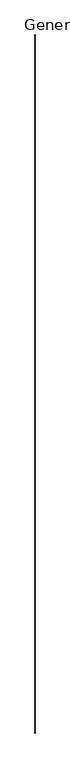
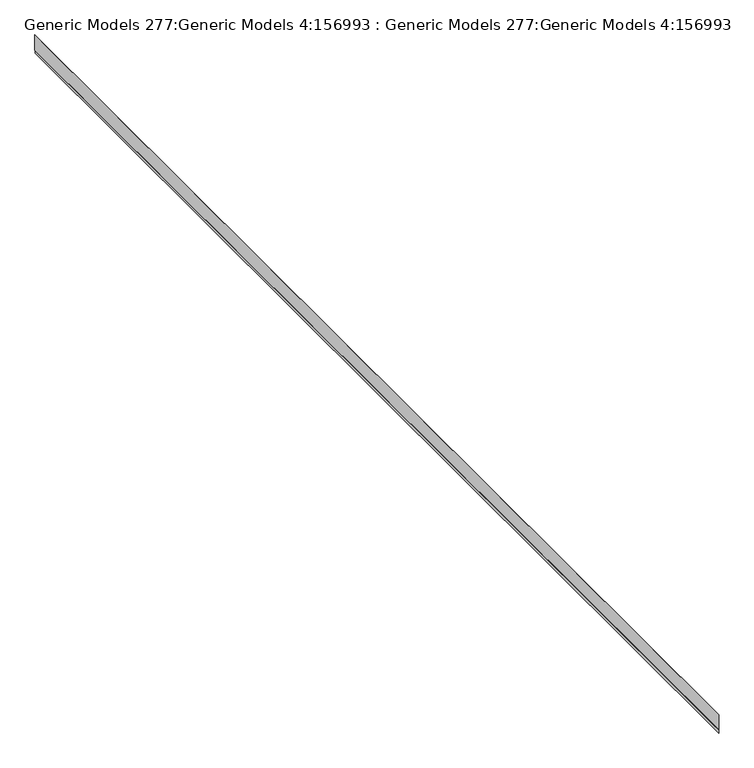
"""IFC4 building model written with IfcOpenShell, lengths in millimetres: proxy geometry, Generic Models 277:Generic Models 4:156993 : Generic Models 277:Generic Models 4:156993."""

import ifcopenshell
import ifcopenshell.guid

model = None  # the IFC model being written
_history = None  # IfcOwnerHistory: only IFC2X3 demands one
_inside = {}  # id of a spatial element -> (the spatial element, [elements in it])
_under = {}  # id of a project, library or spatial element -> (it, [spatial elements below it])
_declared = {}  # id of a project -> (the project, [libraries it declares])
_typed = {}  # id of a type object -> (the type object, [elements of that type])
_made_of = {}  # id of a material, layer set ... -> (it, [elements and type objects made of it])


def new_model(schema):
    """Start an empty IFC model of exactly this schema.

    Asked for "IFC4X3", IfcOpenShell would pick the latest addendum, in which some entities
    have other attributes; the version numbers below select the first issue.
    IFC2X3 requires an IfcOwnerHistory on every rooted entity: one is made here for all.
    """
    global model, _history
    if schema == "IFC4X3":
        model = ifcopenshell.file(schema_version=(4, 3, 0, 0))
    else:
        model = ifcopenshell.file(schema=schema)
    _inside.clear()
    _under.clear()
    _declared.clear()
    _typed.clear()
    _made_of.clear()
    _history = None
    if model.schema == "IFC2X3":
        org = make("IfcOrganization", Name="unknown")
        user = make(
            "IfcPersonAndOrganization",
            ThePerson=make("IfcPerson", FamilyName="unknown"),
            TheOrganization=org,
        )
        app = make(
            "IfcApplication",
            ApplicationDeveloper=org,
            Version="unknown",
            ApplicationFullName="unknown",
            ApplicationIdentifier="unknown",
        )
        _history = make(
            "IfcOwnerHistory",
            OwningUser=user,
            OwningApplication=app,
            ChangeAction="ADDED",
            CreationDate=0,
        )
    return model


def make(cls, **values):
    """One entity of the class cls with the attributes given. An attribute that is None is left unset."""
    return model.create_entity(
        cls, **{name: value for name, value in values.items() if value is not None}
    )


def rooted(cls, **values):
    """An entity with a GlobalId (a new one), such as an element, a storey or a relation."""
    return make(cls, GlobalId=ifcopenshell.guid.new(), OwnerHistory=_history, **values)


def si_unit(unit_type, name, prefix=None):
    """IfcSIUnit, for example si_unit("LENGTHUNIT", "METRE", prefix="MILLI")."""
    return make("IfcSIUnit", UnitType=unit_type, Prefix=prefix, Name=name)


def assignment(units):
    """IfcUnitAssignment: the units of a project."""
    return None if units is None else make("IfcUnitAssignment", Units=units)


def point(xyz):
    """IfcCartesianPoint."""
    return None if xyz is None else make("IfcCartesianPoint", Coordinates=xyz)


def direction(xyz):
    """IfcDirection."""
    return None if xyz is None else make("IfcDirection", DirectionRatios=xyz)


def frame(location, z_axis=None, x_axis=None):
    """IfcAxis2Placement3D, a coordinate frame: its origin and axes. An axis left out is left unset."""
    return make(
        "IfcAxis2Placement3D",
        Location=point(location),
        Axis=direction(z_axis),
        RefDirection=direction(x_axis),
    )


def origin():
    """The frame at (0, 0, 0) with its axes left unset."""
    return frame((0.0, 0.0, 0.0))


def place(relative_to, where):
    """IfcLocalPlacement: puts the frame where relative to a parent placement (None: the world)."""
    return make(
        "IfcLocalPlacement", PlacementRelTo=relative_to, RelativePlacement=where
    )


def context(
    kind, dimensions, precision=None, world=None, true_north=None, identifier=None
):
    """IfcGeometricRepresentationContext, for example the 3D "Model" context."""
    return make(
        "IfcGeometricRepresentationContext",
        ContextIdentifier=identifier,
        ContextType=kind,
        CoordinateSpaceDimension=dimensions,
        Precision=precision,
        WorldCoordinateSystem=world,
        TrueNorth=true_north,
    )


def project(units=None, contexts=None):
    """IfcProject with its units and contexts."""
    return rooted(
        "IfcProject",
        Name="project",
        RepresentationContexts=contexts,
        UnitsInContext=assignment(units),
    )


def spatial(cls, under=None, at=None, **own):
    """A site, building, storey or space (cls), placed at a placement, below another one or the project."""
    s = rooted(cls, ObjectPlacement=at, **own)
    if under is not None:
        _under.setdefault(under.id(), (under, []))[1].append(s)
    return s


def polyline(points):
    """IfcPolyline through the points."""
    return make("IfcPolyline", Points=[point(p) for p in points])


def outline(outer, holes=None, kind="AREA"):
    """IfcArbitraryClosedProfileDef: a profile drawn as a closed curve; with holes, ...WithVoids."""
    if holes is None:
        return make("IfcArbitraryClosedProfileDef", ProfileType=kind, OuterCurve=outer)
    return make(
        "IfcArbitraryProfileDefWithVoids",
        ProfileType=kind,
        OuterCurve=outer,
        InnerCurves=holes,
    )


def extrude(swept, where, along, depth):
    """IfcExtrudedAreaSolid: the profile swept, set in the frame where, extruded along a direction by depth."""
    return make(
        "IfcExtrudedAreaSolid",
        SweptArea=swept,
        Position=where,
        ExtrudedDirection=direction(along),
        Depth=depth,
    )


def shape(context_of_items, identifier, shape_type, items):
    """IfcShapeRepresentation: the items that make up one representation, for example the "Body"."""
    return make(
        "IfcShapeRepresentation",
        ContextOfItems=context_of_items,
        RepresentationIdentifier=identifier,
        RepresentationType=shape_type,
        Items=items,
    )


def source(mapping_origin, context_of_items, identifier, shape_type, items):
    """IfcRepresentationMap: a shape defined once, which mapped items show again and again."""
    return make(
        "IfcRepresentationMap",
        MappingOrigin=mapping_origin,
        MappedRepresentation=shape(context_of_items, identifier, shape_type, items),
    )


def transform(
    local_origin,
    x_axis=None,
    y_axis=None,
    z_axis=None,
    scale=None,
    scale2=None,
    scale3=None,
    uniform=True,
):
    """IfcCartesianTransformationOperator3D, or its non-uniform kind. x_axis, y_axis, z_axis: its Axis1, 2, 3."""
    if uniform:
        return make(
            "IfcCartesianTransformationOperator3D",
            Axis1=direction(x_axis),
            Axis2=direction(y_axis),
            LocalOrigin=point(local_origin),
            Scale=scale,
            Axis3=direction(z_axis),
        )
    return make(
        "IfcCartesianTransformationOperator3DnonUniform",
        Axis1=direction(x_axis),
        Axis2=direction(y_axis),
        LocalOrigin=point(local_origin),
        Scale=scale,
        Axis3=direction(z_axis),
        Scale2=scale2,
        Scale3=scale3,
    )


def mapped(mapping_source, mapping_target):
    """IfcMappedItem: shows the shape of a source again, moved by a transform."""
    return make(
        "IfcMappedItem", MappingSource=mapping_source, MappingTarget=mapping_target
    )


def made_of(thing, what):
    """Note that an element or type object is made of a material, layer set ...; save() writes the relation."""
    if what is not None:
        _made_of.setdefault(what.id(), (what, []))[1].append(thing)
    return thing


def element(
    cls,
    number,
    at=None,
    inside=None,
    cuts=None,
    type_object=None,
    material=None,
    context=None,
    identifier="Body",
    shape_type=None,
    held_by="IfcProductDefinitionShape",
    body=None,
    shapes=None,
    **own,
):
    """One element of the class cls, such as IfcWall. Its Tag is "e" and its number.

    at: its placement. inside: the storey or other place that contains it. cuts: it is an
    opening in that element (IfcRelVoidsElement). A single representation is given by context,
    identifier, shape_type and body (its items); several are given by shapes. held_by: the class
    of the entity that holds the representations. save() writes the other relations.
    """
    e = rooted(cls, Tag="e%d" % number, ObjectPlacement=at, **own)
    if body is not None:
        shapes = [shape(context, identifier, shape_type, body)]
    if shapes is not None:
        e.Representation = make(held_by, Representations=shapes)
    if inside is not None:
        _inside.setdefault(inside.id(), (inside, []))[1].append(e)
    if cuts is not None:
        rooted(
            "IfcRelVoidsElement", RelatingBuildingElement=cuts, RelatedOpeningElement=e
        )
    if type_object is not None:
        _typed.setdefault(type_object.id(), (type_object, []))[1].append(e)
    return made_of(e, material)


def aggregate(whole, parts):
    """IfcRelAggregates: a whole, such as a stair, and the parts it consists of."""
    return rooted("IfcRelAggregates", RelatingObject=whole, RelatedObjects=parts)


def save(model, path):
    """Write the relations noted so far, then the file.

    IfcRelAggregates (storeys below a building ...), IfcRelContainedInSpatialStructure (elements
    in a storey), IfcRelDefinesByType, IfcRelAssociatesMaterial and IfcRelDeclares: one each for
    every whole, place, type object, material and project.
    """
    for whole, parts in _under.values():
        aggregate(whole, parts)
    for where, things in _inside.values():
        rooted(
            "IfcRelContainedInSpatialStructure",
            RelatedElements=things,
            RelatingStructure=where,
        )
    for kind, things in _typed.values():
        rooted("IfcRelDefinesByType", RelatedObjects=things, RelatingType=kind)
    for what, things in _made_of.values():
        rooted("IfcRelAssociatesMaterial", RelatedObjects=things, RelatingMaterial=what)
    for by, libraries in _declared.values():
        rooted("IfcRelDeclares", RelatingContext=by, RelatedDefinitions=libraries)
    model.write(path)


def generic_models_277_generic_models_4_156993_generic_models_47cee2a2(model_context):
    return source(origin(), model_context, "Body", "SweptSolid", [
        extrude(outline(polyline([(6156.5192101, 1597.6373761), (5902.9944211, 1597.6373761), (5897.3527003, 1599.6907945), (5849.785851, 1599.6907945), (5849.785851, 1600.4845445), (5897.4926599, 1600.4845445), (5903.1343806, 1598.4311261), (6156.5192101, 1598.4311261), (6156.5192101, 1597.6373761)])), frame((0.0, -8838.4871142, 0.0), z_axis=(0.0, 1.0, 0.0), x_axis=(0.0, 0.0, 1.0)), (0.0, 0.0, 1.0), 18643.6),
    ])


if __name__ == "__main__":
    model = new_model("IFC4")
    model_context = context("Model", 3, world=origin())
    ifc_project = project(units=[si_unit("LENGTHUNIT", "METRE", prefix="MILLI")], contexts=[model_context])
    site = spatial("IfcSite", under=ifc_project)
    building = spatial("IfcBuilding", under=site)
    placement = place(None, origin())
    generic_models_277_generic_models_4_156993_generic_models_shape = generic_models_277_generic_models_4_156993_generic_models_47cee2a2(model_context)
    element("IfcBuildingElementProxy", 1, Name="Generic Models 277:Generic Models 4:156993 : Generic Models 277:Generic Models 4:156993", ObjectType="Generic Models 277:Generic Models 4:156993 : Generic Models 277:Generic Models 4:156993", at=placement, inside=building, context=model_context, shape_type="MappedRepresentation", body=[
        mapped(generic_models_277_generic_models_4_156993_generic_models_shape, transform((0.0, 0.0, 0.0), x_axis=(1.0, 0.0, 0.0), y_axis=(0.0, 1.0, 0.0), z_axis=(0.0, 0.0, 1.0))),
    ])
    save(model, "model.ifc")

# Revit data of these elements
# Type "Generic Models 277:Generic Models 4:156993 : Generic Models 277:Generic Models 4:156993"
#   NameOverride = "Generic Models 277:Generic Models 4:156993"
#   ObjectTypeOverride = "Generic Models 277:Generic Models 4"
#   Reference = "Generic Models 4"
#   Category = "Generic Models"
#   Tag = "156993"
# Element 1 (IfcBuildingElementProxy, "Generic Models 277:Generic Models 4:156993 : Generic Models 277:Generic Models 4:156993")
#   Materials on its faces: "_DRAINABLE BUILDING WRAP 24696"
# Materials
#   "_DRAINABLE BUILDING WRAP 24696": class "Unassigned", colour RGB 67 154 161, transparency 0
